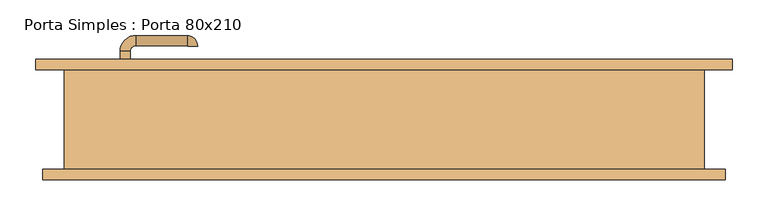
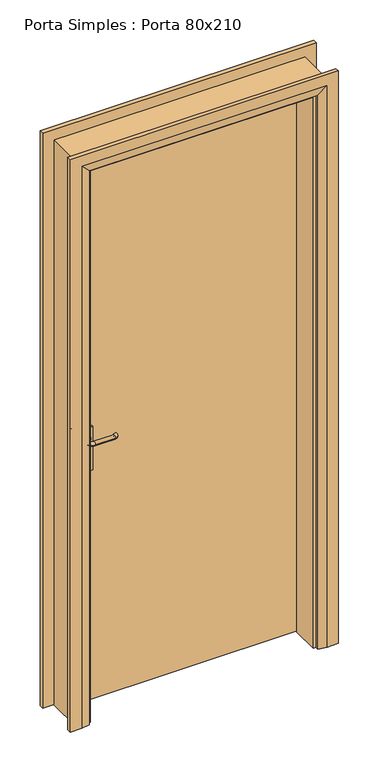
"""IFC4 building model written with IfcOpenShell, lengths in millimetres: door geometry, Porta Simples : Porta 80x210."""

from ifc_helpers import new_model, si_unit, point, frame, frame_2d, origin, place, context, project, spatial, polyline, circle_curve, ellipse_curve, trimmed, segment, composite_curve, outline, extrude, faceted_brep, source, transform, mapped, element, save
from ifc_brep_helpers import plane_surface, cylinder_surface, revolved_surface, advanced_brep


def porta_simples_porta_80x210_f85516ab(model_context):
    return source(origin(), model_context, "Body", "SolidModel", [
        extrude(outline(composite_curve([segment(trimmed(circle_curve(frame_2d((1050.0, -364.0)), 20.0), [point((1050.0, -384.0))], [point((1050.0, -344.0))], False, "CARTESIAN"), True, "CONTINUOUS"), segment(trimmed(circle_curve(frame_2d((1050.0, -364.0)), 20.0), [point((1050.0, -344.0))], [point((1050.0, -384.0))], False, "CARTESIAN"), True, "CONTINUOUS")], self_intersect=False)), frame((0.0, 24.4070105, 0.0), z_axis=(0.0, 1.0, 0.0), x_axis=(0.0, 0.0, 1.0)), (0.0, 0.0, 1.0), 4.5929895),
        advanced_brep(
        [(-357.0, 24.4070105, 1050.0), (-371.0, 24.4070105, 1050.0), (-371.0, 9.0, 1050.0), (-357.0, 9.0, 1050.0), (-349.0, -13.0, 1050.0), (-349.0, 1.0, 1050.0), (-277.0, -13.0, 1050.0), (-277.0, 1.0, 1050.0), (-276.0, 2.0, 1050.0), (-262.0, 2.0, 1050.0)],
        [
            (0, 1, circle_curve(frame((-364.0, 24.4070105, 1050.0), z_axis=(0.0, 1.0, 0.0), x_axis=(-1.0, 0.0, 0.0)), 7.0)),
            (1, 0, circle_curve(frame((-364.0, 24.4070105, 1050.0), z_axis=(0.0, 1.0, 0.0), x_axis=(-1.0, 0.0, 0.0)), 7.0)),
            (1, 2),
            (2, 3, circle_curve(frame((-364.0, 9.0, 1050.0), z_axis=(0.0, 1.0, 0.0), x_axis=(-1.0, 0.0, 0.0)), 7.0)),
            (3, 0),
            (3, 2, circle_curve(frame((-364.0, 9.0, 1050.0), z_axis=(0.0, 1.0, 0.0), x_axis=(-1.0, 0.0, 0.0)), 7.0)),
            (4, 5, circle_curve(frame((-349.0, -6.0, 1050.0), z_axis=(-1.0, 0.0, 0.0), x_axis=(0.0, -1.0, 0.0)), 7.0)),
            (5, 3, circle_curve(frame((-349.0, 9.0, 1050.0), z_axis=(0.0, 0.0, -1.0), x_axis=(-1.0, 0.0, 0.0)), 8.0)),
            (2, 4, circle_curve(frame((-349.0, 9.0, 1050.0), z_axis=(0.0, 0.0, 1.0), x_axis=(-1.0, 0.0, 0.0)), 22.0)),
            (5, 4, circle_curve(frame((-349.0, -6.0, 1050.0), z_axis=(-1.0, 0.0, 0.0), x_axis=(0.0, -1.0, 0.0)), 7.0)),
            (4, 6),
            (6, 7, circle_curve(frame((-277.0, -6.0, 1050.0), z_axis=(-1.0, 0.0, 0.0), x_axis=(0.0, -1.0, 0.0)), 7.0)),
            (7, 5),
            (7, 6, circle_curve(frame((-277.0, -6.0, 1050.0), z_axis=(-1.0, 0.0, 0.0), x_axis=(0.0, -1.0, 0.0)), 7.0)),
            (8, 9, circle_curve(frame((-269.0, 2.0, 1050.0), z_axis=(0.0, 1.0, 0.0), x_axis=(1.0, 0.0, 0.0)), 7.0)),
            (9, 8, circle_curve(frame((-269.0, 2.0, 1050.0), z_axis=(0.0, 1.0, 0.0), x_axis=(1.0, 0.0, 0.0)), 7.0)),
            (8, 7, circle_curve(frame((-277.0, 2.0, 1050.0), z_axis=(0.0, 0.0, -1.0), x_axis=(0.0, -1.0, 0.0)), 1.0)),
            (6, 9, circle_curve(frame((-277.0, 2.0, 1050.0), z_axis=(0.0, 0.0, 1.0), x_axis=(0.0, -1.0, 0.0)), 15.0)),
        ],
        [
            plane_surface(frame((-364.0, 24.4070105, 1050.0), z_axis=(0.0, 1.0, 0.0), x_axis=(0.0, 0.0, 1.0))),
            cylinder_surface(frame((-364.0, 24.4070105, 1050.0), z_axis=(0.0, 1.0, 0.0), x_axis=(-1.0, 0.0, 0.0)), 7.0),
            revolved_surface(trimmed(ellipse_curve(frame((-364.0, 9.0, 1050.0), z_axis=(0.0, -1.0, 0.0), x_axis=(-1.0, 0.0, 0.0)), 7.0, 7.0), [point((-357.0, 9.0, 1050.0))], [point((-371.0, 9.0, 1050.0))], True, "CARTESIAN"), (-349.0, 9.0, 1050.0), (0.0, 0.0, -1.0)),
            revolved_surface(trimmed(ellipse_curve(frame((-364.0, 9.0, 1050.0), z_axis=(0.0, -1.0, 0.0), x_axis=(-1.0, 0.0, 0.0)), 7.0, 7.0), [point((-371.0, 9.0, 1050.0))], [point((-357.0, 9.0, 1050.0))], True, "CARTESIAN"), (-349.0, 9.0, 1050.0), (0.0, 0.0, -1.0)),
            cylinder_surface(frame((-349.0, -6.0, 1050.0), z_axis=(-1.0, 0.0, 0.0), x_axis=(0.0, -1.0, 0.0)), 7.0),
            plane_surface(frame((-269.0, 2.0, 1050.0), z_axis=(0.0, 1.0, 0.0), x_axis=(0.0, 0.0, 1.0))),
            revolved_surface(trimmed(ellipse_curve(frame((-277.0, -6.0, 1050.0), z_axis=(1.0, 0.0, 0.0), x_axis=(0.0, -1.0, 0.0)), 7.0, 7.0), [point((-277.0, 1.0, 1050.0))], [point((-277.0, -13.0, 1050.0))], True, "CARTESIAN"), (-277.0, 2.0, 1050.0), (0.0, 0.0, -1.0)),
            revolved_surface(trimmed(ellipse_curve(frame((-277.0, -6.0, 1050.0), z_axis=(1.0, 0.0, 0.0), x_axis=(0.0, -1.0, 0.0)), 7.0, 7.0), [point((-277.0, -13.0, 1050.0))], [point((-277.0, 1.0, 1050.0))], True, "CARTESIAN"), (-277.0, 2.0, 1050.0), (0.0, 0.0, -1.0)),
        ],
        [
            (0, [[1, 2]]),
            (1, [[3, 4, 5, -2]]),
            (1, [[-5, 6, -3, -1]]),
            (2, [[7, 8, -4, 9]]),
            (3, [[10, -9, -6, -8]]),
            (4, [[11, 12, 13, -7]]),
            (4, [[-13, 14, -11, -10]]),
            (5, [[15, 16]]),
            (6, [[-15, 17, -12, 18]]),
            (7, [[-16, -18, -14, -17]]),
        ],
    ),
        extrude(outline(polyline([(-334.0, 35.0), (-334.0, 29.0), (-394.0, 29.0), (-394.0, 35.0), (-334.0, 35.0)])), frame((0.0, 0.0, 925.0), z_axis=(0.0, 0.0, 1.0), x_axis=(1.0, 0.0, 0.0)), (0.0, 0.0, 1.0), 165.0),
        extrude(outline(composite_curve([segment(trimmed(circle_curve(frame_2d((1050.0, -364.0)), 20.0), [point((1050.0, -384.0))], [point((1050.0, -344.0))], False, "CARTESIAN"), True, "CONTINUOUS"), segment(trimmed(circle_curve(frame_2d((1050.0, -364.0)), 20.0), [point((1050.0, -344.0))], [point((1050.0, -384.0))], False, "CARTESIAN"), True, "CONTINUOUS")], self_intersect=False)), frame((0.0, 76.0, 0.0), z_axis=(0.0, 1.0, 0.0), x_axis=(0.0, 0.0, 1.0)), (0.0, 0.0, 1.0), 4.5929895),
        advanced_brep(
        [(-357.0, 80.5929895, 1050.0), (-371.0, 80.5929895, 1050.0), (-357.0, 96.0, 1050.0), (-371.0, 96.0, 1050.0), (-349.0, 118.0, 1050.0), (-349.0, 104.0, 1050.0), (-277.0, 104.0, 1050.0), (-277.0, 118.0, 1050.0), (-276.0, 103.0, 1050.0), (-262.0, 103.0, 1050.0)],
        [
            (0, 1, circle_curve(frame((-364.0, 80.5929895, 1050.0), z_axis=(0.0, -1.0, 0.0), x_axis=(-1.0, 0.0, 0.0)), 7.0)),
            (1, 0, circle_curve(frame((-364.0, 80.5929895, 1050.0), z_axis=(0.0, -1.0, 0.0), x_axis=(-1.0, 0.0, 0.0)), 7.0)),
            (0, 2),
            (2, 3, circle_curve(frame((-364.0, 96.0, 1050.0), z_axis=(0.0, -1.0, 0.0), x_axis=(-1.0, 0.0, 0.0)), 7.0)),
            (3, 1),
            (3, 2, circle_curve(frame((-364.0, 96.0, 1050.0), z_axis=(0.0, -1.0, 0.0), x_axis=(-1.0, 0.0, 0.0)), 7.0)),
            (4, 3, circle_curve(frame((-349.0, 96.0, 1050.0), z_axis=(0.0, 0.0, 1.0), x_axis=(-1.0, 0.0, 0.0)), 22.0)),
            (2, 5, circle_curve(frame((-349.0, 96.0, 1050.0), z_axis=(0.0, 0.0, -1.0), x_axis=(-1.0, 0.0, 0.0)), 8.0)),
            (5, 4, circle_curve(frame((-349.0, 111.0, 1050.0), z_axis=(-1.0, 0.0, 0.0), x_axis=(0.0, 1.0, 0.0)), 7.0)),
            (4, 5, circle_curve(frame((-349.0, 111.0, 1050.0), z_axis=(-1.0, 0.0, 0.0), x_axis=(0.0, 1.0, 0.0)), 7.0)),
            (5, 6),
            (6, 7, circle_curve(frame((-277.0, 111.0, 1050.0), z_axis=(-1.0, 0.0, 0.0), x_axis=(0.0, 1.0, 0.0)), 7.0)),
            (7, 4),
            (7, 6, circle_curve(frame((-277.0, 111.0, 1050.0), z_axis=(-1.0, 0.0, 0.0), x_axis=(0.0, 1.0, 0.0)), 7.0)),
            (8, 9, circle_curve(frame((-269.0, 103.0, 1050.0), z_axis=(0.0, -1.0, 0.0), x_axis=(1.0, 0.0, 0.0)), 7.0)),
            (9, 8, circle_curve(frame((-269.0, 103.0, 1050.0), z_axis=(0.0, -1.0, 0.0), x_axis=(1.0, 0.0, 0.0)), 7.0)),
            (9, 7, circle_curve(frame((-277.0, 103.0, 1050.0), z_axis=(0.0, 0.0, 1.0), x_axis=(0.0, 1.0, 0.0)), 15.0)),
            (6, 8, circle_curve(frame((-277.0, 103.0, 1050.0), z_axis=(0.0, 0.0, -1.0), x_axis=(0.0, 1.0, 0.0)), 1.0)),
        ],
        [
            plane_surface(frame((-364.0, 80.5929895, 1050.0), z_axis=(0.0, -1.0, 0.0), x_axis=(0.0, 0.0, 1.0))),
            cylinder_surface(frame((-364.0, 80.5929895, 1050.0), z_axis=(0.0, -1.0, 0.0), x_axis=(-1.0, 0.0, 0.0)), 7.0),
            revolved_surface(trimmed(ellipse_curve(frame((-364.0, 96.0, 1050.0), z_axis=(0.0, -1.0, 0.0), x_axis=(-1.0, 0.0, 0.0)), 7.0, 7.0), [point((-357.0, 96.0, 1050.0))], [point((-371.0, 96.0, 1050.0))], True, "CARTESIAN"), (-349.0, 96.0, 1050.0), (0.0, 0.0, -1.0)),
            revolved_surface(trimmed(ellipse_curve(frame((-364.0, 96.0, 1050.0), z_axis=(0.0, -1.0, 0.0), x_axis=(-1.0, 0.0, 0.0)), 7.0, 7.0), [point((-371.0, 96.0, 1050.0))], [point((-357.0, 96.0, 1050.0))], True, "CARTESIAN"), (-349.0, 96.0, 1050.0), (0.0, 0.0, -1.0)),
            cylinder_surface(frame((-349.0, 111.0, 1050.0), z_axis=(-1.0, 0.0, 0.0), x_axis=(0.0, 1.0, 0.0)), 7.0),
            plane_surface(frame((-269.0, 103.0, 1050.0), z_axis=(0.0, -1.0, 0.0), x_axis=(0.0, 0.0, 1.0))),
            revolved_surface(trimmed(ellipse_curve(frame((-277.0, 111.0, 1050.0), z_axis=(-1.0, 0.0, 0.0), x_axis=(0.0, 1.0, 0.0)), 7.0, 7.0), [point((-277.0, 104.0, 1050.0))], [point((-277.0, 118.0, 1050.0))], True, "CARTESIAN"), (-277.0, 103.0, 1050.0), (0.0, 0.0, -1.0)),
            revolved_surface(trimmed(ellipse_curve(frame((-277.0, 111.0, 1050.0), z_axis=(-1.0, 0.0, 0.0), x_axis=(0.0, 1.0, 0.0)), 7.0, 7.0), [point((-277.0, 118.0, 1050.0))], [point((-277.0, 104.0, 1050.0))], True, "CARTESIAN"), (-277.0, 103.0, 1050.0), (0.0, 0.0, -1.0)),
        ],
        [
            (0, [[1, 2]]),
            (1, [[-1, 3, 4, 5]]),
            (1, [[-2, -5, 6, -3]]),
            (2, [[7, -4, 8, 9]]),
            (3, [[-8, -6, -7, 10]]),
            (4, [[-9, 11, 12, 13]]),
            (4, [[-10, -13, 14, -11]]),
            (5, [[15, 16]]),
            (6, [[17, -12, 18, -16]]),
            (7, [[-18, -14, -17, -15]]),
        ],
    ),
        extrude(outline(polyline([(-334.0, 70.0), (-394.0, 70.0), (-394.0, 76.0), (-334.0, 76.0), (-334.0, 70.0)])), frame((0.0, 0.0, 925.0), z_axis=(0.0, 0.0, 1.0), x_axis=(1.0, 0.0, 0.0)), (0.0, 0.0, 1.0), 165.0),
        extrude(outline(polyline([(408.0, 35.0), (-408.0, 35.0), (-408.0, 70.0), (408.0, 70.0), (408.0, 35.0)])), frame((0.0, 0.0, 53.0), z_axis=(0.0, 0.0, 1.0), x_axis=(1.0, 0.0, 0.0)), (0.0, 0.0, 1.0), 2094.0),
        faceted_brep([(480.0, -70.0, 50.0), (480.0, -85.0, 50.0), (440.0, -85.0, 50.0), (410.0, -80.0, 50.0), (410.0, -70.0, 50.0), (480.0, -70.0, 2220.0), (480.0, -85.0, 2220.0), (-480.0, -85.0, 2220.0), (-480.0, -85.0, 50.0), (-440.0, -85.0, 50.0), (-440.0, -85.0, 2180.0), (440.0, -85.0, 2180.0), (410.0, -80.0, 2150.0), (410.0, -70.0, 2150.0), (-410.0, -70.0, 2150.0), (-410.0, -70.0, 50.0), (-480.0, -70.0, 50.0), (-480.0, -70.0, 2220.0), (-410.0, -80.0, 2150.0), (-410.0, -80.0, 50.0)], [[[0, 1, 2, 3, 4]], [[1, 0, 5, 6]], [[2, 1, 6, 7, 8, 9, 10, 11]], [[3, 2, 11, 12]], [[4, 3, 12, 13]], [[0, 4, 13, 14, 15, 16, 17, 5]], [[14, 18, 19, 15]], [[16, 15, 19, 9, 8]], [[7, 17, 16, 8]], [[18, 10, 9, 19]], [[13, 12, 18, 14]], [[6, 5, 17, 7]], [[12, 11, 10, 18]]]),
        faceted_brep([(490.0, 70.0, 50.0), (420.0, 70.0, 50.0), (420.0, 80.0, 50.0), (450.0, 85.0, 50.0), (490.0, 85.0, 50.0), (490.0, 70.0, 2230.0), (-490.0, 70.0, 2230.0), (-490.0, 70.0, 50.0), (-420.0, 70.0, 50.0), (-420.0, 70.0, 2160.0), (420.0, 70.0, 2160.0), (420.0, 80.0, 2160.0), (450.0, 85.0, 2190.0), (-450.0, 85.0, 2190.0), (-450.0, 85.0, 50.0), (-490.0, 85.0, 50.0), (-490.0, 85.0, 2230.0), (490.0, 85.0, 2230.0), (-420.0, 80.0, 50.0), (-420.0, 80.0, 2160.0)], [[[0, 1, 2, 3, 4]], [[1, 0, 5, 6, 7, 8, 9, 10]], [[2, 1, 10, 11]], [[3, 2, 11, 12]], [[4, 3, 12, 13, 14, 15, 16, 17]], [[0, 4, 17, 5]], [[6, 16, 15, 7]], [[7, 15, 14, 18, 8]], [[19, 9, 8, 18]], [[13, 19, 18, 14]], [[11, 10, 9, 19]], [[5, 17, 16, 6]], [[12, 11, 19, 13]]]),
        faceted_brep([(-410.0, 70.0, 50.0), (-410.0, 33.0, 50.0), (-400.0, 33.0, 50.0), (-400.0, -70.0, 50.0), (-450.0, -70.0, 50.0), (-450.0, 70.0, 50.0), (-410.0, 70.0, 2150.0), (-410.0, 33.0, 2150.0), (-400.0, 33.0, 2140.0), (-400.0, -70.0, 2140.0), (-450.0, -70.0, 2190.0), (-450.0, 70.0, 2190.0), (410.0, 70.0, 50.0), (450.0, 70.0, 50.0), (450.0, -70.0, 50.0), (400.0, -70.0, 50.0), (400.0, 33.0, 50.0), (410.0, 33.0, 50.0), (410.0, 70.0, 2150.0), (450.0, 70.0, 2190.0), (450.0, -70.0, 2190.0), (400.0, -70.0, 2140.0), (400.0, 33.0, 2140.0), (410.0, 33.0, 2150.0)], [[[0, 1, 2, 3, 4, 5]], [[1, 0, 6, 7]], [[2, 1, 7, 8]], [[3, 2, 8, 9]], [[4, 3, 9, 10]], [[5, 4, 10, 11]], [[0, 5, 11, 6]], [[12, 13, 14, 15, 16, 17]], [[18, 19, 13, 12]], [[19, 20, 14, 13]], [[20, 21, 15, 14]], [[21, 22, 16, 15]], [[22, 23, 17, 16]], [[23, 18, 12, 17]], [[7, 6, 18, 23]], [[8, 7, 23, 22]], [[9, 8, 22, 21]], [[10, 9, 21, 20]], [[11, 10, 20, 19]], [[6, 11, 19, 18]]]),
    ])


if __name__ == "__main__":
    model = new_model("IFC4")
    model_context = context("Model", 3, world=origin())
    ifc_project = project(units=[si_unit("LENGTHUNIT", "METRE", prefix="MILLI")], contexts=[model_context])
    site = spatial("IfcSite", under=ifc_project)
    building = spatial("IfcBuilding", under=site)
    placement = place(None, origin())
    porta_simples_porta_80x210_shape = porta_simples_porta_80x210_f85516ab(model_context)
    element("IfcDoor", 1, ObjectType="Porta Simples : Porta 80x210", at=placement, inside=building, context=model_context, shape_type="MappedRepresentation", body=[
        mapped(porta_simples_porta_80x210_shape, transform((0.0, 0.0, 0.0), x_axis=(1.0, 0.0, 0.0), y_axis=(0.0, 1.0, 0.0), z_axis=(0.0, 0.0, 1.0))),
    ])
    save(model, "model.ifc")

# Revit data of these elements
# Type "Porta Simples : Porta 80x210"
#   Type Mark = "49"
#   SINAPI = ""
#   Analytic Construction = "<Nenhum>"
#   Construction Type = "300"
#   Maçaneta [instance default] = ""
#   Fechadura [instance default] = ""
#   Vão Luz (somente para informação) = 0.78 m
#   Tolerância Folha Vertical = 0.003 m
#   Módulo Básico M = 0.10 m
#   Largura de Coordenação Modular Largura CM = 0.90 m
#   Rough Width = 0.90 m
#   Deslocamento da Horizontal da Folha = 0.00 m
#   Altura de Coordenação Modular Largura CM = 2.20 m
#   Rough Height = 2.20 m
#   Altura Nominal = 2.09 m
#   Ajuste de Coordenação Topo AC Topo = 0.01 m
#   Ajuste de Coordenação Base AC Base = 0.05 m
#   Ajuste de Coordenação AC = 0.01 m
#   Tolerância Folha Horizontal = 0.002 m
#   Largura Folha (somente para informação) = 0.796 m
#   Espessura Folha = 0.035 m
#   Maçaneta - Distância da Folha = 0.044 m
#   Maçaneta - Altura = 1.00 m
#   Largura Nominal (Largura Mn) = 0.82 m
#   Distância do Nível = 0.003 m
#   Aduela Interna Espessura = 0.04 m
#   Aduela Externa Espessura = 0.05 m
#   Altura Folha (somente para informação) = 2.075 m
#   Height = 2.14 m
#   Width = 0.88 m
#   Número de Módulos Básicos nM Largura = 9
#   Número de Módulos Básicos nM Altura = 22
#   Marco Metálico = no
#   Aduela de Madeira = no
#   Aduela Metálica de Canto = no
#   Guarnição Reta = no
#   Guarnição Chanfrada = yes
#   Batente - Material [instance default] = none
#   Painel - Material [instance default] = none
#   Model = ""
#   Function = (empty or 0)
#   Description = (empty or 0)
#   Wall Closure = (empty or 0)
#   Assembly Code = ""
# Element 1 (IfcDoor, "Porta Simples : Porta 80x210")
#   Materials on its faces: "Porta - Maçaneta"
# Materials
#   "Porta - Maçaneta": class "Diversos", colour RGB 0 0 0, transparency 0
